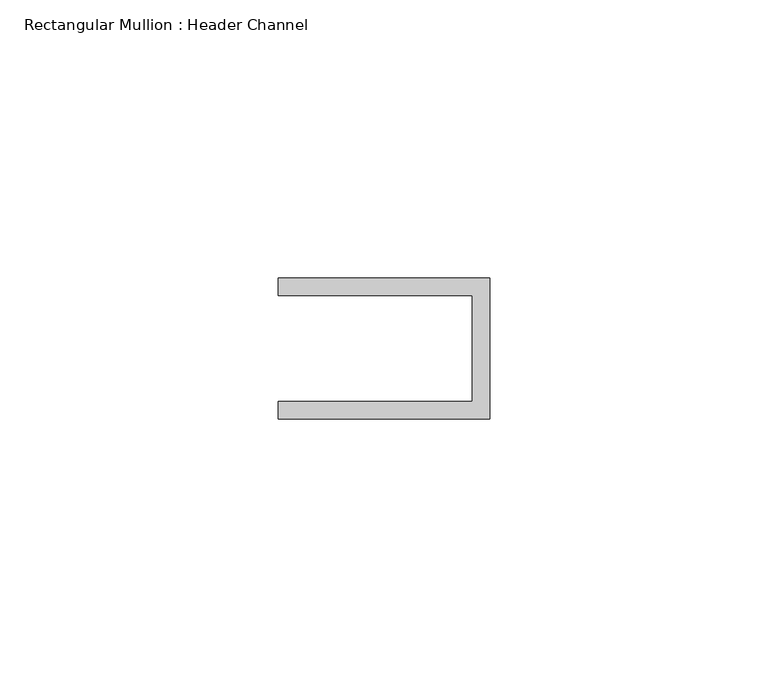
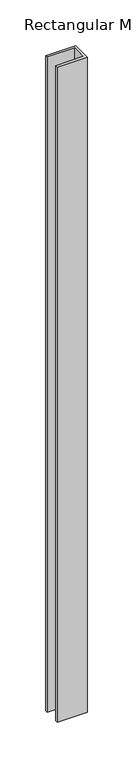
"""IFC4 building model written with IfcOpenShell, lengths in millimetres: member geometry, Rectangular Mullion : Header Channel."""

from ifc_helpers import new_model, si_unit, frame, origin, place, context, project, spatial, polyline, outline, extrude, source, transform, mapped, element, save


def rectangular_mullion_header_channel_a2631777(model_context):
    return source(origin(), model_context, "Body", "SweptSolid", [
        extrude(outline(polyline([(0.0, -12.7), (-38.1, -12.7), (-38.1, -9.525), (-3.175, -9.525), (-3.175, 9.525), (-38.1, 9.525), (-38.1, 12.7), (0.0, 12.7), (0.0, -12.7)])), frame((0.0, 0.0, -877.8332392), z_axis=(0.0, 0.0, 1.0), x_axis=(1.0, 0.0, 0.0)), (0.0, 0.0, 1.0), 877.8332392),
    ])


if __name__ == "__main__":
    model = new_model("IFC4")
    model_context = context("Model", 3, world=origin())
    ifc_project = project(units=[si_unit("LENGTHUNIT", "METRE", prefix="MILLI")], contexts=[model_context])
    site = spatial("IfcSite", under=ifc_project)
    building = spatial("IfcBuilding", under=site)
    placement = place(None, origin())
    rectangular_mullion_header_channel_shape = rectangular_mullion_header_channel_a2631777(model_context)
    element("IfcMember", 1, ObjectType="Rectangular Mullion : Header Channel", at=placement, inside=building, context=model_context, shape_type="MappedRepresentation", body=[
        mapped(rectangular_mullion_header_channel_shape, transform((0.0, 0.0, 0.0), x_axis=(1.0, 0.0, 0.0), y_axis=(0.0, 1.0, 0.0), z_axis=(0.0, 0.0, 1.0))),
    ])
    save(model, "model.ifc")

# Revit data of these elements
# Type "Rectangular Mullion : Header Channel"
#   built-in parameter 1007322 = 0.0833333 (stored number, unit not read)
#   built-in parameter 1007321 = -0.03125 (stored number, unit not read)
#   built-in parameter 1007320 = 0.0416667 (stored number, unit not read)
# Element 1 (IfcMember, "Rectangular Mullion : Header Channel")
#   Materials on its faces: "ALUM"
# Materials
#   "ALUM": class "Generic", colour RGB 157 157 157, transparency 0, Cost = 0
